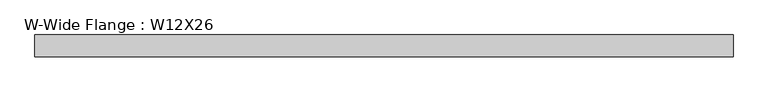
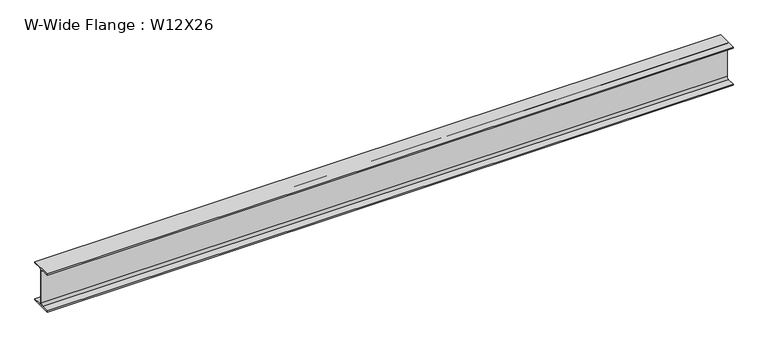
"""IFC4 building model written with IfcOpenShell, lengths in millimetres: beam geometry, W-Wide Flange : W12X26."""

from ifc_helpers import new_model, si_unit, point, frame, frame_2d, origin, place, context, project, spatial, polyline, circle_curve, trimmed, segment, composite_curve, outline, extrude, source, transform, mapped, element, save


def w_wide_flange_w12x26_6f15523d(model_context):
    return source(origin(), model_context, "Body", "SweptSolid", [
        extrude(outline(composite_curve([segment(polyline([(82.4011719, -145.5539063), (82.4011719, -155.178125), (-82.4011719, -155.178125), (-82.4011719, -145.5539063), (-20.2902344, -145.5539063)]), True, "CONTINUOUS"), segment(trimmed(circle_curve(frame_2d((-20.2902344, -128.190625)), 17.3632812), [point((-20.2902344, -145.5539063))], [point((-2.9269531, -128.190625))], True, "CARTESIAN"), True, "CONTINUOUS"), segment(polyline([(-2.9269531, -128.190625), (-2.9269531, 128.190625)]), True, "CONTINUOUS"), segment(trimmed(circle_curve(frame_2d((-20.2902344, 128.190625)), 17.3632812), [point((-2.9269531, 128.190625))], [point((-20.2902344, 145.5539062))], True, "CARTESIAN"), True, "CONTINUOUS"), segment(polyline([(-20.2902344, 145.5539062), (-82.4011719, 145.5539062), (-82.4011719, 155.178125), (82.4011719, 155.178125), (82.4011719, 145.5539062), (20.2902344, 145.5539062)]), True, "CONTINUOUS"), segment(trimmed(circle_curve(frame_2d((20.2902344, 128.190625)), 17.3632812), [point((20.2902344, 145.5539062))], [point((2.9269531, 128.190625))], True, "CARTESIAN"), True, "CONTINUOUS"), segment(polyline([(2.9269531, 128.190625), (2.9269531, -128.190625)]), True, "CONTINUOUS"), segment(trimmed(circle_curve(frame_2d((20.2902344, -128.190625)), 17.3632812), [point((2.9269531, -128.190625))], [point((20.2902344, -145.5539063))], True, "CARTESIAN"), True, "CONTINUOUS"), segment(polyline([(20.2902344, -145.5539063), (82.4011719, -145.5539063)]), True, "CONTINUOUS")], self_intersect=False)), frame((-2633.8467178, 0.0, 0.0), z_axis=(1.0, 0.0, 0.0), x_axis=(0.0, 1.0, 0.0)), (0.0, 0.0, 1.0), 5267.6934356),
    ])


if __name__ == "__main__":
    model = new_model("IFC4")
    model_context = context("Model", 3, world=origin())
    ifc_project = project(units=[si_unit("LENGTHUNIT", "METRE", prefix="MILLI")], contexts=[model_context])
    site = spatial("IfcSite", under=ifc_project)
    building = spatial("IfcBuilding", under=site)
    placement = place(None, origin())
    w_wide_flange_w12x26_shape = w_wide_flange_w12x26_6f15523d(model_context)
    element("IfcBeam", 1, ObjectType="W-Wide Flange : W12X26", at=placement, inside=building, context=model_context, shape_type="MappedRepresentation", body=[
        mapped(w_wide_flange_w12x26_shape, transform((0.0, 0.0, 0.0), x_axis=(1.0, 0.0, 0.0), y_axis=(0.0, 1.0, 0.0), z_axis=(0.0, 0.0, 1.0))),
    ])
    save(model, "model.ifc")

# Revit data of these elements
# Type "W-Wide Flange : W12X26"
#   Assembly Code = "B10"
#   W = 26
#   Length [instance default] = 5' - 0"
#   bf = 0' - 6 125/256"
#   d = 1' - 0 7/32"
#   k = 0' - 1 1/16"
#   k2 = 0' - 0 175/256"
#   tf = 0' - 0 97/256"
#   tw = 0' - 0 59/256"
#   A = 0.053125 SF
#   Structural Material [instance default] = Steel ASTM A992
# Element 1 (IfcBeam, "W-Wide Flange : W12X26")
#   Structural Material = STRUCTURAL STEEL - SEE STRUCT. DWGS
#   Materials on its faces: "STRUCTURAL STEEL - SEE STRUCT. DWGS"
# Materials
#   "Steel ASTM A992": class "Metal", colour RGB 199 199 199, transparency 0, Description = "Structural steel 50ksi", Cost = 0
#   "STRUCTURAL STEEL - SEE STRUCT. DWGS": class "Metal", colour RGB 137 146 153, transparency 0, Description = "Steel, mill finish", Cost = 0
